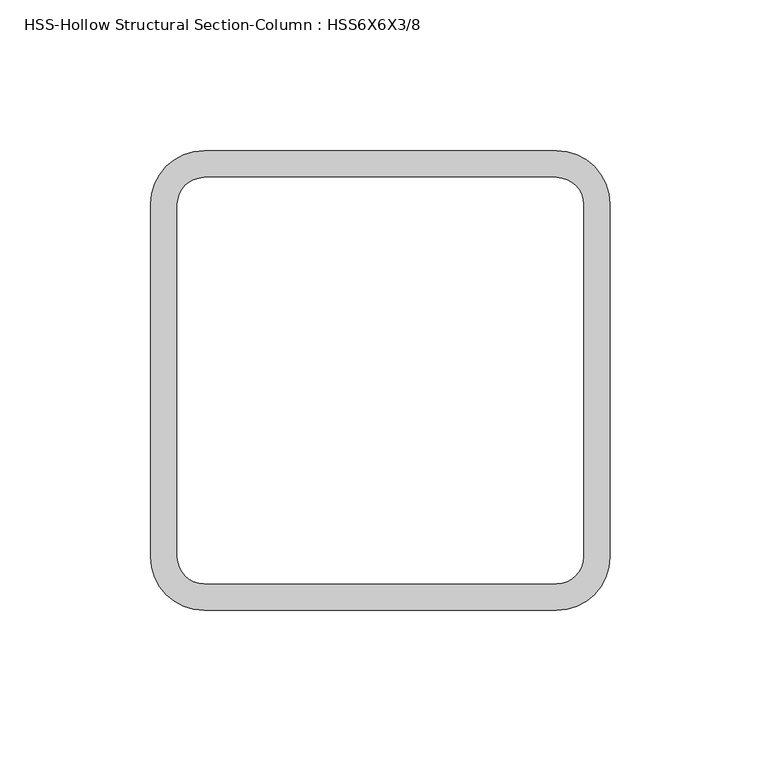
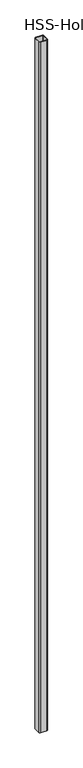
"""IFC4 building model written with IfcOpenShell, lengths in millimetres: column geometry, HSS-Hollow Structural Section-Column : HSS6X6X3/8."""

from ifc_helpers import new_model, si_unit, point, frame, frame_2d, origin, place, context, project, spatial, polyline, circle_curve, trimmed, segment, composite_curve, outline, extrude, source, transform, mapped, element, save


def hss_hollow_structural_section_column_hss6x6x3_8_d99481d2(model_context):
    return source(origin(), model_context, "Body", "SweptSolid", [
        extrude(outline(composite_curve([segment(trimmed(circle_curve(frame_2d((58.4708, 58.4708)), 17.7292), [point((58.4708, 76.2))], [point((76.2, 58.4708))], False, "CARTESIAN"), True, "CONTINUOUS"), segment(polyline([(76.2, 58.4708), (76.2, -58.4708)]), True, "CONTINUOUS"), segment(trimmed(circle_curve(frame_2d((58.4708, -58.4708)), 17.7292), [point((76.2, -58.4708))], [point((58.4708, -76.2))], False, "CARTESIAN"), True, "CONTINUOUS"), segment(polyline([(58.4708, -76.2), (-58.4708, -76.2)]), True, "CONTINUOUS"), segment(trimmed(circle_curve(frame_2d((-58.4708, -58.4708)), 17.7292), [point((-58.4708, -76.2))], [point((-76.2, -58.4708))], False, "CARTESIAN"), True, "CONTINUOUS"), segment(polyline([(-76.2, -58.4708), (-76.2, 58.4708)]), True, "CONTINUOUS"), segment(trimmed(circle_curve(frame_2d((-58.4708, 58.4708)), 17.7292), [point((-76.2, 58.4708))], [point((-58.4708, 76.2))], False, "CARTESIAN"), True, "CONTINUOUS"), segment(polyline([(-58.4708, 76.2), (58.4708, 76.2)]), True, "CONTINUOUS")], self_intersect=False), holes=[composite_curve([segment(polyline([(58.4708, 67.3354), (-58.4708, 67.3354)]), True, "CONTINUOUS"), segment(trimmed(circle_curve(frame_2d((-58.4708, 58.4708)), 8.8646), [point((-58.4708, 67.3354))], [point((-67.3354, 58.4708))], True, "CARTESIAN"), True, "CONTINUOUS"), segment(polyline([(-67.3354, 58.4708), (-67.3354, -58.4708)]), True, "CONTINUOUS"), segment(trimmed(circle_curve(frame_2d((-58.4708, -58.4708)), 8.8646), [point((-67.3354, -58.4708))], [point((-58.4708, -67.3354))], True, "CARTESIAN"), True, "CONTINUOUS"), segment(polyline([(-58.4708, -67.3354), (58.4708, -67.3354)]), True, "CONTINUOUS"), segment(trimmed(circle_curve(frame_2d((58.4708, -58.4708)), 8.8646), [point((58.4708, -67.3354))], [point((67.3354, -58.4708))], True, "CARTESIAN"), True, "CONTINUOUS"), segment(polyline([(67.3354, -58.4708), (67.3354, 58.4708)]), True, "CONTINUOUS"), segment(trimmed(circle_curve(frame_2d((58.4708, 58.4708)), 8.8646), [point((67.3354, 58.4708))], [point((58.4708, 67.3354))], True, "CARTESIAN"), True, "CONTINUOUS")], self_intersect=False)]), frame((0.0, 0.0, -609.6), z_axis=(0.0, 0.0, 1.0), x_axis=(1.0, 0.0, 0.0)), (0.0, 0.0, 1.0), 13157.2),
    ])


if __name__ == "__main__":
    model = new_model("IFC4")
    model_context = context("Model", 3, world=origin())
    ifc_project = project(units=[si_unit("LENGTHUNIT", "METRE", prefix="MILLI")], contexts=[model_context])
    site = spatial("IfcSite", under=ifc_project)
    building = spatial("IfcBuilding", under=site)
    placement = place(None, origin())
    hss_hollow_structural_section_column_hss6x6x3_8_shape = hss_hollow_structural_section_column_hss6x6x3_8_d99481d2(model_context)
    element("IfcColumn", 1, ObjectType="HSS-Hollow Structural Section-Column : HSS6X6X3/8", at=placement, inside=building, context=model_context, shape_type="MappedRepresentation", body=[
        mapped(hss_hollow_structural_section_column_hss6x6x3_8_shape, transform((0.0, 0.0, 0.0), x_axis=(1.0, 0.0, 0.0), y_axis=(0.0, 1.0, 0.0), z_axis=(0.0, 0.0, 1.0))),
    ])
    save(model, "model.ifc")

# Revit data of these elements
# Type "HSS-Hollow Structural Section-Column : HSS6X6X3/8"
#   Assembly Code = "B10"
#   Shape = "Square"
#   W = 27.4
#   Ht = 0' - 6"
#   b = 0' - 6"
#   kr = 0' - 0.698"
#   t = 0' - 0.349"
#   A = 0.0526389 SF
#   Structural Material [instance default] = Steel ASTM A500, Grade B, Rectangular and Square
# Element 1 (IfcColumn, "HSS-Hollow Structural Section-Column : HSS6X6X3/8")
#   Materials on its faces: "Steel ASTM A500, Grade B, Rectangular and Square"
# Materials
#   "Steel ASTM A500, Grade B, Rectangular and Square": class "Metal", colour RGB 199 199 199, transparency 0, Description = "Carbon steel", Cost = 0
